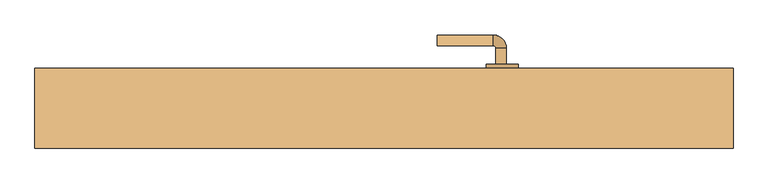
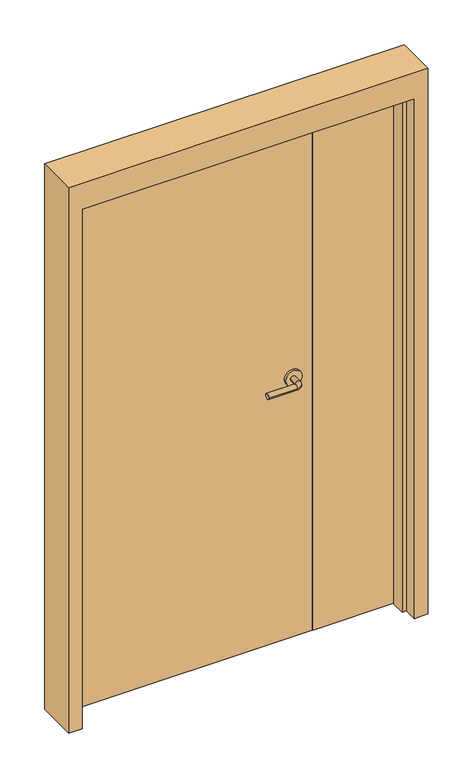
"""IFC4 building model written with IfcOpenShell, lengths in millimetres: door geometry, Дверь-Маятниковая-С полотнами разной ширины-Щитовая : 1310 x 2100 мм."""

from ifc_helpers import new_model, si_unit, point, frame, frame_2d, origin, origin_with_axes, place, context, project, spatial, polyline, circle_curve, ellipse_curve, trimmed, segment, composite_curve, outline, extrude, faceted_brep, source, transform, mapped, element, save
from ifc_brep_helpers import plane_surface, cylinder_surface, revolved_surface, advanced_brep


def door_dc542a90(model_context):
    return source(origin(), model_context, "Body", "SolidModel", [
        advanced_brep(
        [(229.59375, 3.35, 1000.0), (209.59375, 3.35, 1000.0), (229.59375, -26.65, 1000.0), (209.59375, -26.65, 1000.0), (204.59375, -31.65, 1000.0), (204.59375, -51.65, 1000.0), (99.59375, -51.65, 1000.0), (99.59375, -31.65, 1000.0)],
        [
            (0, 1, circle_curve(frame((219.59375, 3.35, 1000.0), z_axis=(0.0, 1.0, 0.0), x_axis=(-1.0, 0.0, 0.0)), 10.0)),
            (1, 0, circle_curve(frame((219.59375, 3.35, 1000.0), z_axis=(0.0, 1.0, 0.0), x_axis=(-1.0, 0.0, 0.0)), 10.0)),
            (0, 2),
            (2, 3, circle_curve(frame((219.59375, -26.65, 1000.0), z_axis=(0.0, 1.0, 0.0), x_axis=(-1.0, 0.0, 0.0)), 10.0)),
            (3, 1),
            (3, 2, circle_curve(frame((219.59375, -26.65, 1000.0), z_axis=(0.0, 1.0, 0.0), x_axis=(-1.0, 0.0, 0.0)), 10.0)),
            (4, 3, circle_curve(frame((204.59375, -26.65, 1000.0), z_axis=(0.0, 0.0, 1.0), x_axis=(1.0, 0.0, 0.0)), 5.0)),
            (2, 5, circle_curve(frame((204.59375, -26.65, 1000.0), z_axis=(0.0, 0.0, -1.0), x_axis=(1.0, 0.0, 0.0)), 25.0)),
            (5, 4, circle_curve(frame((204.59375, -41.65, 1000.0), z_axis=(1.0, 0.0, 0.0), x_axis=(0.0, 1.0, 0.0)), 10.0)),
            (4, 5, circle_curve(frame((204.59375, -41.65, 1000.0), z_axis=(1.0, 0.0, 0.0), x_axis=(0.0, 1.0, 0.0)), 10.0)),
            (6, 7, circle_curve(frame((99.59375, -41.65, 1000.0), z_axis=(-1.0, 0.0, 0.0), x_axis=(0.0, 1.0, 0.0)), 10.0)),
            (7, 6, circle_curve(frame((99.59375, -41.65, 1000.0), z_axis=(-1.0, 0.0, 0.0), x_axis=(0.0, 1.0, 0.0)), 10.0)),
            (5, 6),
            (7, 4),
        ],
        [
            plane_surface(frame((219.59375, 3.35, 1000.0), z_axis=(0.0, 1.0, 0.0), x_axis=(0.0, 0.0, 1.0))),
            cylinder_surface(frame((219.59375, 3.35, 1000.0), z_axis=(0.0, 1.0, 0.0), x_axis=(-1.0, 0.0, 0.0)), 10.0),
            revolved_surface(trimmed(ellipse_curve(frame((219.59375, -26.65, 1000.0), z_axis=(0.0, 1.0, 0.0), x_axis=(-1.0, 0.0, 0.0)), 10.0, 10.0), [point((229.59375, -26.65, 1000.0))], [point((209.59375, -26.65, 1000.0))], True, "CARTESIAN"), (204.59375, -26.65, 1000.0), (0.0, 0.0, -1.0)),
            revolved_surface(trimmed(ellipse_curve(frame((219.59375, -26.65, 1000.0), z_axis=(0.0, 1.0, 0.0), x_axis=(-1.0, 0.0, 0.0)), 10.0, 10.0), [point((209.59375, -26.65, 1000.0))], [point((229.59375, -26.65, 1000.0))], True, "CARTESIAN"), (204.59375, -26.65, 1000.0), (0.0, 0.0, -1.0)),
            plane_surface(frame((99.59375, -41.65, 1000.0), z_axis=(-1.0, 0.0, 0.0), x_axis=(0.0, 0.0, 1.0))),
            cylinder_surface(frame((204.59375, -41.65, 1000.0), z_axis=(1.0, 0.0, 0.0), x_axis=(0.0, 1.0, 0.0)), 10.0),
        ],
        [
            (0, [[1, 2]]),
            (1, [[-1, 3, 4, 5]]),
            (1, [[-2, -5, 6, -3]]),
            (2, [[7, -4, 8, 9]]),
            (3, [[-8, -6, -7, 10]]),
            (4, [[11, 12]]),
            (5, [[-9, 13, -12, 14]]),
            (5, [[-10, -14, -11, -13]]),
        ],
    ),
        extrude(outline(composite_curve([segment(trimmed(circle_curve(frame_2d((1000.0, 222.09375)), 30.0), [point((1000.0, 252.09375))], [point((1000.0, 192.09375))], False, "CARTESIAN"), True, "CONTINUOUS"), segment(trimmed(circle_curve(frame_2d((1000.0, 222.09375)), 30.0), [point((1000.0, 192.09375))], [point((1000.0, 252.09375))], False, "CARTESIAN"), True, "CONTINUOUS")], self_intersect=False)), frame((0.0, 3.35, 0.0), z_axis=(0.0, 1.0, 0.0), x_axis=(0.0, 0.0, 1.0)), (0.0, 0.0, 1.0), 8.0),
        advanced_brep(
        [(229.59375, 64.35, 1000.0), (209.59375, 64.35, 1000.0), (209.59375, 94.35, 1000.0), (229.59375, 94.35, 1000.0), (204.59375, 99.35, 1000.0), (204.59375, 119.35, 1000.0), (99.59375, 119.35, 1000.0), (99.59375, 99.35, 1000.0)],
        [
            (0, 1, circle_curve(frame((219.59375, 64.35, 1000.0), z_axis=(0.0, -1.0, 0.0), x_axis=(-1.0, 0.0, 0.0)), 10.0)),
            (1, 0, circle_curve(frame((219.59375, 64.35, 1000.0), z_axis=(0.0, -1.0, 0.0), x_axis=(-1.0, 0.0, 0.0)), 10.0)),
            (1, 2),
            (2, 3, circle_curve(frame((219.59375, 94.35, 1000.0), z_axis=(0.0, -1.0, 0.0), x_axis=(-1.0, 0.0, 0.0)), 10.0)),
            (3, 0),
            (3, 2, circle_curve(frame((219.59375, 94.35, 1000.0), z_axis=(0.0, -1.0, 0.0), x_axis=(-1.0, 0.0, 0.0)), 10.0)),
            (4, 5, circle_curve(frame((204.59375, 109.35, 1000.0), z_axis=(1.0, 0.0, 0.0), x_axis=(0.0, -1.0, 0.0)), 10.0)),
            (5, 3, circle_curve(frame((204.59375, 94.35, 1000.0), z_axis=(0.0, 0.0, -1.0), x_axis=(1.0, 0.0, 0.0)), 25.0)),
            (2, 4, circle_curve(frame((204.59375, 94.35, 1000.0), z_axis=(0.0, 0.0, 1.0), x_axis=(1.0, 0.0, 0.0)), 5.0)),
            (5, 4, circle_curve(frame((204.59375, 109.35, 1000.0), z_axis=(1.0, 0.0, 0.0), x_axis=(0.0, -1.0, 0.0)), 10.0)),
            (6, 7, circle_curve(frame((99.59375, 109.35, 1000.0), z_axis=(-1.0, 0.0, 0.0), x_axis=(0.0, -1.0, 0.0)), 10.0)),
            (7, 6, circle_curve(frame((99.59375, 109.35, 1000.0), z_axis=(-1.0, 0.0, 0.0), x_axis=(0.0, -1.0, 0.0)), 10.0)),
            (4, 7),
            (6, 5),
        ],
        [
            plane_surface(frame((219.59375, 64.35, 1000.0), z_axis=(0.0, -1.0, 0.0), x_axis=(0.0, 0.0, 1.0))),
            cylinder_surface(frame((219.59375, 64.35, 1000.0), z_axis=(0.0, -1.0, 0.0), x_axis=(-1.0, 0.0, 0.0)), 10.0),
            revolved_surface(trimmed(ellipse_curve(frame((219.59375, 94.35, 1000.0), z_axis=(0.0, 1.0, 0.0), x_axis=(-1.0, 0.0, 0.0)), 10.0, 10.0), [point((229.59375, 94.35, 1000.0))], [point((209.59375, 94.35, 1000.0))], True, "CARTESIAN"), (204.59375, 94.35, 1000.0), (0.0, 0.0, -1.0)),
            revolved_surface(trimmed(ellipse_curve(frame((219.59375, 94.35, 1000.0), z_axis=(0.0, 1.0, 0.0), x_axis=(-1.0, 0.0, 0.0)), 10.0, 10.0), [point((209.59375, 94.35, 1000.0))], [point((229.59375, 94.35, 1000.0))], True, "CARTESIAN"), (204.59375, 94.35, 1000.0), (0.0, 0.0, -1.0)),
            plane_surface(frame((99.59375, 109.35, 1000.0), z_axis=(-1.0, 0.0, 0.0), x_axis=(0.0, 0.0, 1.0))),
            cylinder_surface(frame((204.59375, 109.35, 1000.0), z_axis=(1.0, 0.0, 0.0), x_axis=(0.0, -1.0, 0.0)), 10.0),
        ],
        [
            (0, [[1, 2]]),
            (1, [[3, 4, 5, -2]]),
            (1, [[-5, 6, -3, -1]]),
            (2, [[7, 8, -4, 9]]),
            (3, [[10, -9, -6, -8]]),
            (4, [[11, 12]]),
            (5, [[13, -11, 14, -7]]),
            (5, [[-14, -12, -13, -10]]),
        ],
    ),
        extrude(outline(composite_curve([segment(trimmed(circle_curve(frame_2d((1000.0, 222.09375)), 30.0), [point((1000.0, 252.09375))], [point((1000.0, 192.09375))], False, "CARTESIAN"), True, "CONTINUOUS"), segment(trimmed(circle_curve(frame_2d((1000.0, 222.09375)), 30.0), [point((1000.0, 192.09375))], [point((1000.0, 252.09375))], False, "CARTESIAN"), True, "CONTINUOUS")], self_intersect=False)), frame((0.0, 56.35, 0.0), z_axis=(0.0, 1.0, 0.0), x_axis=(0.0, 0.0, 1.0)), (0.0, 0.0, 1.0), 8.0),
        extrude(outline(polyline([(605.0, 11.35), (296.6, 11.35), (296.6, 56.35), (605.0, 56.35), (605.0, 11.35)])), origin_with_axes(), (0.0, 0.0, 1.0), 2000.0),
        faceted_brep([(605.0, 6.5875, 0.0), (605.0, 56.35, 0.0), (655.0, 56.35, 0.0), (655.0, -93.65, 0.0), (605.0, -93.65, 0.0), (605.0, -44.4375, 0.0), (589.125, -44.4375, 0.0), (589.125, 6.5875, 0.0), (605.0, 6.5875, 2000.0), (605.0, 56.35, 2000.0), (-605.0, 56.35, 2000.0), (-605.0, 56.35, 0.0), (-655.0, 56.35, 0.0), (-655.0, 56.35, 2100.0), (655.0, 56.35, 2100.0), (655.0, -93.65, 2100.0), (-655.0, -93.65, 2100.0), (-655.0, -93.65, 0.0), (-605.0, -93.65, 0.0), (-605.0, -93.65, 2000.0), (605.0, -93.65, 2000.0), (605.0, -44.4375, 2000.0), (-605.0, -44.4375, 2000.0), (-605.0, -44.4375, 0.0), (-589.125, -44.4375, 0.0), (-589.125, -44.4375, 1984.125), (589.125, -44.4375, 1984.125), (589.125, 6.5875, 1984.125), (-589.125, 6.5875, 1984.125), (-589.125, 6.5875, 0.0), (-605.0, 6.5875, 0.0), (-605.0, 6.5875, 2000.0)], [[[0, 1, 2, 3, 4, 5, 6, 7]], [[1, 0, 8, 9]], [[2, 1, 9, 10, 11, 12, 13, 14]], [[3, 2, 14, 15]], [[4, 3, 15, 16, 17, 18, 19, 20]], [[5, 4, 20, 21]], [[6, 5, 21, 22, 23, 24, 25, 26]], [[7, 6, 26, 27]], [[0, 7, 27, 28, 29, 30, 31, 8]], [[9, 8, 31, 10]], [[20, 19, 22, 21]], [[26, 25, 28, 27]], [[12, 11, 30, 29, 24, 23, 18, 17]], [[11, 10, 31, 30]], [[13, 12, 17, 16]], [[19, 18, 23, 22]], [[25, 24, 29, 28]], [[15, 14, 13, 16]]]),
        extrude(outline(polyline([(293.4, 11.35), (-605.0, 11.35), (-605.0, 56.35), (293.4, 56.35), (293.4, 11.35)])), origin_with_axes(), (0.0, 0.0, 1.0), 2000.0),
    ])


if __name__ == "__main__":
    model = new_model("IFC4")
    model_context = context("Model", 3, world=origin())
    ifc_project = project(units=[si_unit("LENGTHUNIT", "METRE", prefix="MILLI")], contexts=[model_context])
    site = spatial("IfcSite", under=ifc_project)
    building = spatial("IfcBuilding", under=site)
    placement = place(None, origin())
    door_shape = door_dc542a90(model_context)
    element("IfcDoor", 1, ObjectType="Дверь-Маятниковая-С полотнами разной ширины-Щитовая : 1310 x 2100 мм", at=placement, inside=building, context=model_context, shape_type="MappedRepresentation", body=[
        mapped(door_shape, transform((0.0, 0.0, 0.0), x_axis=(1.0, 0.0, 0.0), y_axis=(0.0, 1.0, 0.0), z_axis=(0.0, 0.0, 1.0))),
    ])
    save(model, "model.ifc")

# Revit data of these elements
# Type "Дверь-Маятниковая-С полотнами разной ширины-Щитовая : 1310 x 2100 мм"
#   Type Mark = "150"
#   Assembly Code = "C1020300"
#   Analytic Construction = "Деревянный"
#   Ширина большой панели = 900 mm
#   W = 310 mm
#   Thickness = 45 mm
#   Thermal Resistance (R) = 0.455703 (m²·K)/W
#   Угол поворота [instance default] = 90°
#   Высота планки = 1000 mm
#   Rough Width [instance default] = 1310 mm
#   Rough Height [instance default] = 2100 mm
#   Высота проема в кирпичном каркасе [instance default] = 100 mm
#   Ширина проема в кирпичном каркасе [instance default] = 100 mm
#   Расчет вставки [instance default] = 105 mm
#   Кирпичная вставка [instance default] = 25 mm
#   Height = 2000 mm
#   Width = 1210 mm
#   Heat Transfer Coefficient (U) = 2.19465 W/(m²·K)
#   Глубина кирпичного каркаса = 150 mm
#   Кирпичный каркас [instance default] = yes
#   Каркас стены сухой кладки [instance default] = no
#   Материал панели = Древесина - Береза
#   Материал каркаса = Металл - Окрашенный - Серый 2
#   Материал дверной ручки = Алюминий
#   Visual Light Transmittance = 0
#   Solar Heat Gain Coefficient = 0
#   Wall Closure = (empty or 0)
#   Function = (empty or 0)
# Element 1 (IfcDoor, "Дверь-Маятниковая-С полотнами разной ширины-Щитовая : 1310 x 2100 мм")
#   Materials on its faces: "Алюминий", "Металл - Окрашенный - Серый 2", "Древесина - Береза"
# Materials
#   "Древесина - Береза": class "Древесина", colour RGB 166 116 52, transparency 0, Cost = 0
#   "Металл - Окрашенный - Серый 2": class "Краска", colour RGB 104 104 104, transparency 0, Cost = 0
#   "Алюминий": class "Металл", colour RGB 247 247 247, transparency 0
